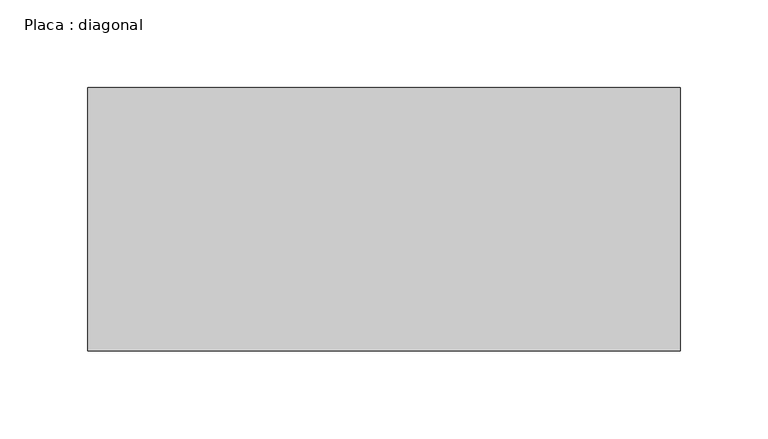
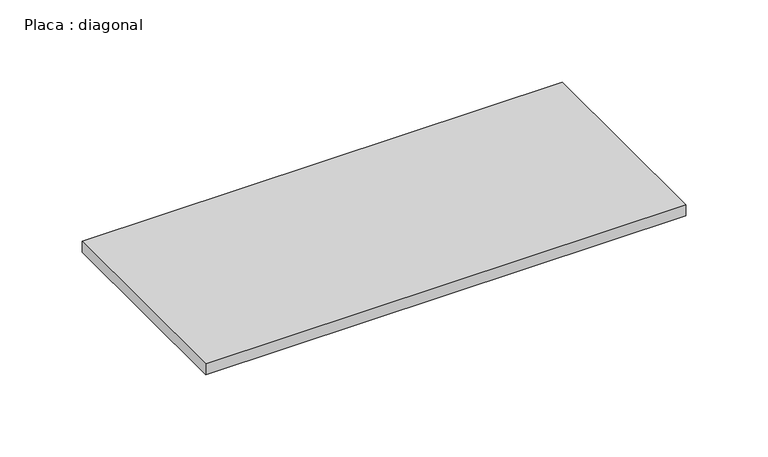
"""IFC4 building model written with IfcOpenShell, lengths in millimetres: beam geometry, Placa : diagonal."""

from ifc_helpers import new_model, si_unit, frame, origin, place, context, project, spatial, polyline, outline, extrude, source, transform, mapped, element, save


def placa_diagonal_854ad00f(model_context):
    return source(origin(), model_context, "Body", "SweptSolid", [
        extrude(outline(polyline([(168.6204795, 75.0), (168.6204795, -75.0), (-168.6204795, -75.0), (-168.6204795, 75.0), (168.6204795, 75.0)])), frame((0.0, 0.0, -4.0), z_axis=(0.0, 0.0, 1.0), x_axis=(1.0, 0.0, 0.0)), (0.0, 0.0, 1.0), 8.0),
    ])


if __name__ == "__main__":
    model = new_model("IFC4")
    model_context = context("Model", 3, world=origin())
    ifc_project = project(units=[si_unit("LENGTHUNIT", "METRE", prefix="MILLI")], contexts=[model_context])
    site = spatial("IfcSite", under=ifc_project)
    building = spatial("IfcBuilding", under=site)
    placement = place(None, origin())
    placa_diagonal_shape = placa_diagonal_854ad00f(model_context)
    element("IfcBeam", 1, ObjectType="Placa : diagonal", at=placement, inside=building, context=model_context, shape_type="MappedRepresentation", body=[
        mapped(placa_diagonal_shape, transform((0.0, 0.0, 0.0), x_axis=(1.0, 0.0, 0.0), y_axis=(0.0, 1.0, 0.0), z_axis=(0.0, 0.0, 1.0))),
    ])
    save(model, "model.ifc")

# Revit data of these elements
# Type "Placa : diagonal"
#   W = 0
#   Length [instance default] = 1.50 m
#   b = 0.15 m
#   d = 0.008 m
#   A = 0 m²
#   Structural Material [instance default] = Aço, 45-345
# Element 1 (IfcBeam, "Placa : diagonal")
#   Materials on its faces: "Aço, 45-345"
# Materials
#   "Aço, 45-345": class "Metal", colour RGB 247 247 247, transparency 0, Description = "Aço 345 MPa", Cost = 0
